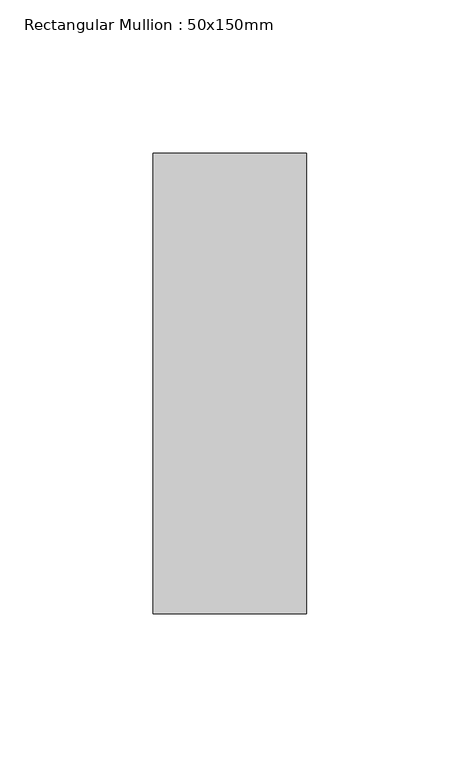
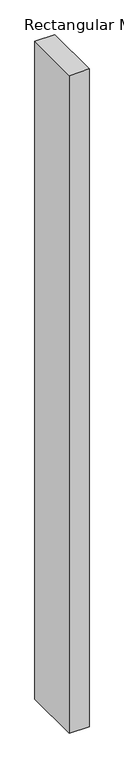
"""IFC4 building model written with IfcOpenShell, lengths in millimetres: member geometry, Rectangular Mullion : 50x150mm."""

import ifcopenshell
import ifcopenshell.guid

model = None  # the IFC model being written
_history = None  # IfcOwnerHistory: only IFC2X3 demands one
_inside = {}  # id of a spatial element -> (the spatial element, [elements in it])
_under = {}  # id of a project, library or spatial element -> (it, [spatial elements below it])
_declared = {}  # id of a project -> (the project, [libraries it declares])
_typed = {}  # id of a type object -> (the type object, [elements of that type])
_made_of = {}  # id of a material, layer set ... -> (it, [elements and type objects made of it])


def new_model(schema):
    """Start an empty IFC model of exactly this schema.

    Asked for "IFC4X3", IfcOpenShell would pick the latest addendum, in which some entities
    have other attributes; the version numbers below select the first issue.
    IFC2X3 requires an IfcOwnerHistory on every rooted entity: one is made here for all.
    """
    global model, _history
    if schema == "IFC4X3":
        model = ifcopenshell.file(schema_version=(4, 3, 0, 0))
    else:
        model = ifcopenshell.file(schema=schema)
    _inside.clear()
    _under.clear()
    _declared.clear()
    _typed.clear()
    _made_of.clear()
    _history = None
    if model.schema == "IFC2X3":
        org = make("IfcOrganization", Name="unknown")
        user = make(
            "IfcPersonAndOrganization",
            ThePerson=make("IfcPerson", FamilyName="unknown"),
            TheOrganization=org,
        )
        app = make(
            "IfcApplication",
            ApplicationDeveloper=org,
            Version="unknown",
            ApplicationFullName="unknown",
            ApplicationIdentifier="unknown",
        )
        _history = make(
            "IfcOwnerHistory",
            OwningUser=user,
            OwningApplication=app,
            ChangeAction="ADDED",
            CreationDate=0,
        )
    return model


def make(cls, **values):
    """One entity of the class cls with the attributes given. An attribute that is None is left unset."""
    return model.create_entity(
        cls, **{name: value for name, value in values.items() if value is not None}
    )


def rooted(cls, **values):
    """An entity with a GlobalId (a new one), such as an element, a storey or a relation."""
    return make(cls, GlobalId=ifcopenshell.guid.new(), OwnerHistory=_history, **values)


def si_unit(unit_type, name, prefix=None):
    """IfcSIUnit, for example si_unit("LENGTHUNIT", "METRE", prefix="MILLI")."""
    return make("IfcSIUnit", UnitType=unit_type, Prefix=prefix, Name=name)


def assignment(units):
    """IfcUnitAssignment: the units of a project."""
    return None if units is None else make("IfcUnitAssignment", Units=units)


def point(xyz):
    """IfcCartesianPoint."""
    return None if xyz is None else make("IfcCartesianPoint", Coordinates=xyz)


def direction(xyz):
    """IfcDirection."""
    return None if xyz is None else make("IfcDirection", DirectionRatios=xyz)


def frame(location, z_axis=None, x_axis=None):
    """IfcAxis2Placement3D, a coordinate frame: its origin and axes. An axis left out is left unset."""
    return make(
        "IfcAxis2Placement3D",
        Location=point(location),
        Axis=direction(z_axis),
        RefDirection=direction(x_axis),
    )


def origin():
    """The frame at (0, 0, 0) with its axes left unset."""
    return frame((0.0, 0.0, 0.0))


def place(relative_to, where):
    """IfcLocalPlacement: puts the frame where relative to a parent placement (None: the world)."""
    return make(
        "IfcLocalPlacement", PlacementRelTo=relative_to, RelativePlacement=where
    )


def context(
    kind, dimensions, precision=None, world=None, true_north=None, identifier=None
):
    """IfcGeometricRepresentationContext, for example the 3D "Model" context."""
    return make(
        "IfcGeometricRepresentationContext",
        ContextIdentifier=identifier,
        ContextType=kind,
        CoordinateSpaceDimension=dimensions,
        Precision=precision,
        WorldCoordinateSystem=world,
        TrueNorth=true_north,
    )


def project(units=None, contexts=None):
    """IfcProject with its units and contexts."""
    return rooted(
        "IfcProject",
        Name="project",
        RepresentationContexts=contexts,
        UnitsInContext=assignment(units),
    )


def spatial(cls, under=None, at=None, **own):
    """A site, building, storey or space (cls), placed at a placement, below another one or the project."""
    s = rooted(cls, ObjectPlacement=at, **own)
    if under is not None:
        _under.setdefault(under.id(), (under, []))[1].append(s)
    return s


def polyline(points):
    """IfcPolyline through the points."""
    return make("IfcPolyline", Points=[point(p) for p in points])


def outline(outer, holes=None, kind="AREA"):
    """IfcArbitraryClosedProfileDef: a profile drawn as a closed curve; with holes, ...WithVoids."""
    if holes is None:
        return make("IfcArbitraryClosedProfileDef", ProfileType=kind, OuterCurve=outer)
    return make(
        "IfcArbitraryProfileDefWithVoids",
        ProfileType=kind,
        OuterCurve=outer,
        InnerCurves=holes,
    )


def extrude(swept, where, along, depth):
    """IfcExtrudedAreaSolid: the profile swept, set in the frame where, extruded along a direction by depth."""
    return make(
        "IfcExtrudedAreaSolid",
        SweptArea=swept,
        Position=where,
        ExtrudedDirection=direction(along),
        Depth=depth,
    )


def shape(context_of_items, identifier, shape_type, items):
    """IfcShapeRepresentation: the items that make up one representation, for example the "Body"."""
    return make(
        "IfcShapeRepresentation",
        ContextOfItems=context_of_items,
        RepresentationIdentifier=identifier,
        RepresentationType=shape_type,
        Items=items,
    )


def source(mapping_origin, context_of_items, identifier, shape_type, items):
    """IfcRepresentationMap: a shape defined once, which mapped items show again and again."""
    return make(
        "IfcRepresentationMap",
        MappingOrigin=mapping_origin,
        MappedRepresentation=shape(context_of_items, identifier, shape_type, items),
    )


def transform(
    local_origin,
    x_axis=None,
    y_axis=None,
    z_axis=None,
    scale=None,
    scale2=None,
    scale3=None,
    uniform=True,
):
    """IfcCartesianTransformationOperator3D, or its non-uniform kind. x_axis, y_axis, z_axis: its Axis1, 2, 3."""
    if uniform:
        return make(
            "IfcCartesianTransformationOperator3D",
            Axis1=direction(x_axis),
            Axis2=direction(y_axis),
            LocalOrigin=point(local_origin),
            Scale=scale,
            Axis3=direction(z_axis),
        )
    return make(
        "IfcCartesianTransformationOperator3DnonUniform",
        Axis1=direction(x_axis),
        Axis2=direction(y_axis),
        LocalOrigin=point(local_origin),
        Scale=scale,
        Axis3=direction(z_axis),
        Scale2=scale2,
        Scale3=scale3,
    )


def mapped(mapping_source, mapping_target):
    """IfcMappedItem: shows the shape of a source again, moved by a transform."""
    return make(
        "IfcMappedItem", MappingSource=mapping_source, MappingTarget=mapping_target
    )


def made_of(thing, what):
    """Note that an element or type object is made of a material, layer set ...; save() writes the relation."""
    if what is not None:
        _made_of.setdefault(what.id(), (what, []))[1].append(thing)
    return thing


def element(
    cls,
    number,
    at=None,
    inside=None,
    cuts=None,
    type_object=None,
    material=None,
    context=None,
    identifier="Body",
    shape_type=None,
    held_by="IfcProductDefinitionShape",
    body=None,
    shapes=None,
    **own,
):
    """One element of the class cls, such as IfcWall. Its Tag is "e" and its number.

    at: its placement. inside: the storey or other place that contains it. cuts: it is an
    opening in that element (IfcRelVoidsElement). A single representation is given by context,
    identifier, shape_type and body (its items); several are given by shapes. held_by: the class
    of the entity that holds the representations. save() writes the other relations.
    """
    e = rooted(cls, Tag="e%d" % number, ObjectPlacement=at, **own)
    if body is not None:
        shapes = [shape(context, identifier, shape_type, body)]
    if shapes is not None:
        e.Representation = make(held_by, Representations=shapes)
    if inside is not None:
        _inside.setdefault(inside.id(), (inside, []))[1].append(e)
    if cuts is not None:
        rooted(
            "IfcRelVoidsElement", RelatingBuildingElement=cuts, RelatedOpeningElement=e
        )
    if type_object is not None:
        _typed.setdefault(type_object.id(), (type_object, []))[1].append(e)
    return made_of(e, material)


def aggregate(whole, parts):
    """IfcRelAggregates: a whole, such as a stair, and the parts it consists of."""
    return rooted("IfcRelAggregates", RelatingObject=whole, RelatedObjects=parts)


def save(model, path):
    """Write the relations noted so far, then the file.

    IfcRelAggregates (storeys below a building ...), IfcRelContainedInSpatialStructure (elements
    in a storey), IfcRelDefinesByType, IfcRelAssociatesMaterial and IfcRelDeclares: one each for
    every whole, place, type object, material and project.
    """
    for whole, parts in _under.values():
        aggregate(whole, parts)
    for where, things in _inside.values():
        rooted(
            "IfcRelContainedInSpatialStructure",
            RelatedElements=things,
            RelatingStructure=where,
        )
    for kind, things in _typed.values():
        rooted("IfcRelDefinesByType", RelatedObjects=things, RelatingType=kind)
    for what, things in _made_of.values():
        rooted("IfcRelAssociatesMaterial", RelatedObjects=things, RelatingMaterial=what)
    for by, libraries in _declared.values():
        rooted("IfcRelDeclares", RelatingContext=by, RelatedDefinitions=libraries)
    model.write(path)


def rectangular_mullion_50x150mm_df7bd136(model_context):
    return source(origin(), model_context, "Body", "SweptSolid", [
        extrude(outline(polyline([(25.0, 75.0), (25.0, -75.0), (-25.0, -75.0), (-25.0, 75.0), (25.0, 75.0)])), frame((0.0, 0.0, -1755.0), z_axis=(0.0, 0.0, 1.0), x_axis=(1.0, 0.0, 0.0)), (0.0, 0.0, 1.0), 1755.0),
    ])


if __name__ == "__main__":
    model = new_model("IFC4")
    model_context = context("Model", 3, world=origin())
    ifc_project = project(units=[si_unit("LENGTHUNIT", "METRE", prefix="MILLI")], contexts=[model_context])
    site = spatial("IfcSite", under=ifc_project)
    building = spatial("IfcBuilding", under=site)
    placement = place(None, origin())
    rectangular_mullion_50x150mm_shape = rectangular_mullion_50x150mm_df7bd136(model_context)
    element("IfcMember", 1, ObjectType="Rectangular Mullion : 50x150mm", at=placement, inside=building, context=model_context, shape_type="MappedRepresentation", body=[
        mapped(rectangular_mullion_50x150mm_shape, transform((0.0, 0.0, 0.0), x_axis=(1.0, 0.0, 0.0), y_axis=(0.0, 1.0, 0.0), z_axis=(0.0, 0.0, 1.0))),
    ])
    save(model, "model.ifc")

# Revit data of these elements
# Type "Rectangular Mullion : 50x150mm"
#   Keynote = "H11"
#   built-in parameter 1007304 = 0.492126 (stored number, unit not read)
#   built-in parameter 1007301 = 0.082021 (stored number, unit not read)
#   built-in parameter 1007300 = 0.082021 (stored number, unit not read)
# Element 1 (IfcMember, "Rectangular Mullion : 50x150mm")
#   Materials on its faces: "Aluminium"
# Materials
#   "Aluminium": class "Metal", colour RGB 247 247 247, transparency 0, Description = "Aluminium 6061", Cost = 0
